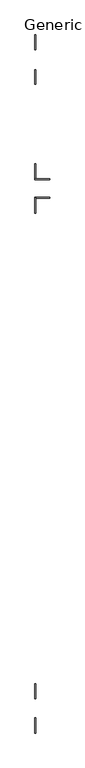
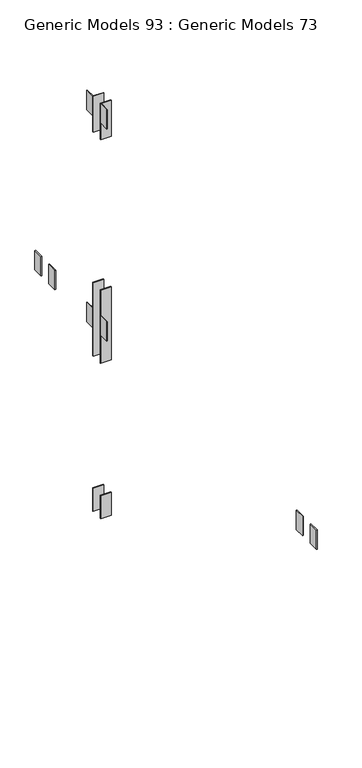
"""IFC4 building model written with IfcOpenShell, lengths in millimetres: proxy geometry, Generic Models 93 : Generic Models 73."""

import ifcopenshell
import ifcopenshell.guid

model = None  # the IFC model being written
_history = None  # IfcOwnerHistory: only IFC2X3 demands one
_inside = {}  # id of a spatial element -> (the spatial element, [elements in it])
_under = {}  # id of a project, library or spatial element -> (it, [spatial elements below it])
_declared = {}  # id of a project -> (the project, [libraries it declares])
_typed = {}  # id of a type object -> (the type object, [elements of that type])
_made_of = {}  # id of a material, layer set ... -> (it, [elements and type objects made of it])


def new_model(schema):
    """Start an empty IFC model of exactly this schema.

    Asked for "IFC4X3", IfcOpenShell would pick the latest addendum, in which some entities
    have other attributes; the version numbers below select the first issue.
    IFC2X3 requires an IfcOwnerHistory on every rooted entity: one is made here for all.
    """
    global model, _history
    if schema == "IFC4X3":
        model = ifcopenshell.file(schema_version=(4, 3, 0, 0))
    else:
        model = ifcopenshell.file(schema=schema)
    _inside.clear()
    _under.clear()
    _declared.clear()
    _typed.clear()
    _made_of.clear()
    _history = None
    if model.schema == "IFC2X3":
        org = make("IfcOrganization", Name="unknown")
        user = make(
            "IfcPersonAndOrganization",
            ThePerson=make("IfcPerson", FamilyName="unknown"),
            TheOrganization=org,
        )
        app = make(
            "IfcApplication",
            ApplicationDeveloper=org,
            Version="unknown",
            ApplicationFullName="unknown",
            ApplicationIdentifier="unknown",
        )
        _history = make(
            "IfcOwnerHistory",
            OwningUser=user,
            OwningApplication=app,
            ChangeAction="ADDED",
            CreationDate=0,
        )
    return model


def make(cls, **values):
    """One entity of the class cls with the attributes given. An attribute that is None is left unset."""
    return model.create_entity(
        cls, **{name: value for name, value in values.items() if value is not None}
    )


def rooted(cls, **values):
    """An entity with a GlobalId (a new one), such as an element, a storey or a relation."""
    return make(cls, GlobalId=ifcopenshell.guid.new(), OwnerHistory=_history, **values)


def si_unit(unit_type, name, prefix=None):
    """IfcSIUnit, for example si_unit("LENGTHUNIT", "METRE", prefix="MILLI")."""
    return make("IfcSIUnit", UnitType=unit_type, Prefix=prefix, Name=name)


def assignment(units):
    """IfcUnitAssignment: the units of a project."""
    return None if units is None else make("IfcUnitAssignment", Units=units)


def point(xyz):
    """IfcCartesianPoint."""
    return None if xyz is None else make("IfcCartesianPoint", Coordinates=xyz)


def direction(xyz):
    """IfcDirection."""
    return None if xyz is None else make("IfcDirection", DirectionRatios=xyz)


def frame(location, z_axis=None, x_axis=None):
    """IfcAxis2Placement3D, a coordinate frame: its origin and axes. An axis left out is left unset."""
    return make(
        "IfcAxis2Placement3D",
        Location=point(location),
        Axis=direction(z_axis),
        RefDirection=direction(x_axis),
    )


def origin():
    """The frame at (0, 0, 0) with its axes left unset."""
    return frame((0.0, 0.0, 0.0))


def place(relative_to, where):
    """IfcLocalPlacement: puts the frame where relative to a parent placement (None: the world)."""
    return make(
        "IfcLocalPlacement", PlacementRelTo=relative_to, RelativePlacement=where
    )


def context(
    kind, dimensions, precision=None, world=None, true_north=None, identifier=None
):
    """IfcGeometricRepresentationContext, for example the 3D "Model" context."""
    return make(
        "IfcGeometricRepresentationContext",
        ContextIdentifier=identifier,
        ContextType=kind,
        CoordinateSpaceDimension=dimensions,
        Precision=precision,
        WorldCoordinateSystem=world,
        TrueNorth=true_north,
    )


def project(units=None, contexts=None):
    """IfcProject with its units and contexts."""
    return rooted(
        "IfcProject",
        Name="project",
        RepresentationContexts=contexts,
        UnitsInContext=assignment(units),
    )


def spatial(cls, under=None, at=None, **own):
    """A site, building, storey or space (cls), placed at a placement, below another one or the project."""
    s = rooted(cls, ObjectPlacement=at, **own)
    if under is not None:
        _under.setdefault(under.id(), (under, []))[1].append(s)
    return s


def polyline(points):
    """IfcPolyline through the points."""
    return make("IfcPolyline", Points=[point(p) for p in points])


def outline(outer, holes=None, kind="AREA"):
    """IfcArbitraryClosedProfileDef: a profile drawn as a closed curve; with holes, ...WithVoids."""
    if holes is None:
        return make("IfcArbitraryClosedProfileDef", ProfileType=kind, OuterCurve=outer)
    return make(
        "IfcArbitraryProfileDefWithVoids",
        ProfileType=kind,
        OuterCurve=outer,
        InnerCurves=holes,
    )


def extrude(swept, where, along, depth):
    """IfcExtrudedAreaSolid: the profile swept, set in the frame where, extruded along a direction by depth."""
    return make(
        "IfcExtrudedAreaSolid",
        SweptArea=swept,
        Position=where,
        ExtrudedDirection=direction(along),
        Depth=depth,
    )


def shape(context_of_items, identifier, shape_type, items):
    """IfcShapeRepresentation: the items that make up one representation, for example the "Body"."""
    return make(
        "IfcShapeRepresentation",
        ContextOfItems=context_of_items,
        RepresentationIdentifier=identifier,
        RepresentationType=shape_type,
        Items=items,
    )


def source(mapping_origin, context_of_items, identifier, shape_type, items):
    """IfcRepresentationMap: a shape defined once, which mapped items show again and again."""
    return make(
        "IfcRepresentationMap",
        MappingOrigin=mapping_origin,
        MappedRepresentation=shape(context_of_items, identifier, shape_type, items),
    )


def transform(
    local_origin,
    x_axis=None,
    y_axis=None,
    z_axis=None,
    scale=None,
    scale2=None,
    scale3=None,
    uniform=True,
):
    """IfcCartesianTransformationOperator3D, or its non-uniform kind. x_axis, y_axis, z_axis: its Axis1, 2, 3."""
    if uniform:
        return make(
            "IfcCartesianTransformationOperator3D",
            Axis1=direction(x_axis),
            Axis2=direction(y_axis),
            LocalOrigin=point(local_origin),
            Scale=scale,
            Axis3=direction(z_axis),
        )
    return make(
        "IfcCartesianTransformationOperator3DnonUniform",
        Axis1=direction(x_axis),
        Axis2=direction(y_axis),
        LocalOrigin=point(local_origin),
        Scale=scale,
        Axis3=direction(z_axis),
        Scale2=scale2,
        Scale3=scale3,
    )


def mapped(mapping_source, mapping_target):
    """IfcMappedItem: shows the shape of a source again, moved by a transform."""
    return make(
        "IfcMappedItem", MappingSource=mapping_source, MappingTarget=mapping_target
    )


def made_of(thing, what):
    """Note that an element or type object is made of a material, layer set ...; save() writes the relation."""
    if what is not None:
        _made_of.setdefault(what.id(), (what, []))[1].append(thing)
    return thing


def element(
    cls,
    number,
    at=None,
    inside=None,
    cuts=None,
    type_object=None,
    material=None,
    context=None,
    identifier="Body",
    shape_type=None,
    held_by="IfcProductDefinitionShape",
    body=None,
    shapes=None,
    **own,
):
    """One element of the class cls, such as IfcWall. Its Tag is "e" and its number.

    at: its placement. inside: the storey or other place that contains it. cuts: it is an
    opening in that element (IfcRelVoidsElement). A single representation is given by context,
    identifier, shape_type and body (its items); several are given by shapes. held_by: the class
    of the entity that holds the representations. save() writes the other relations.
    """
    e = rooted(cls, Tag="e%d" % number, ObjectPlacement=at, **own)
    if body is not None:
        shapes = [shape(context, identifier, shape_type, body)]
    if shapes is not None:
        e.Representation = make(held_by, Representations=shapes)
    if inside is not None:
        _inside.setdefault(inside.id(), (inside, []))[1].append(e)
    if cuts is not None:
        rooted(
            "IfcRelVoidsElement", RelatingBuildingElement=cuts, RelatedOpeningElement=e
        )
    if type_object is not None:
        _typed.setdefault(type_object.id(), (type_object, []))[1].append(e)
    return made_of(e, material)


def aggregate(whole, parts):
    """IfcRelAggregates: a whole, such as a stair, and the parts it consists of."""
    return rooted("IfcRelAggregates", RelatingObject=whole, RelatedObjects=parts)


def save(model, path):
    """Write the relations noted so far, then the file.

    IfcRelAggregates (storeys below a building ...), IfcRelContainedInSpatialStructure (elements
    in a storey), IfcRelDefinesByType, IfcRelAssociatesMaterial and IfcRelDeclares: one each for
    every whole, place, type object, material and project.
    """
    for whole, parts in _under.values():
        aggregate(whole, parts)
    for where, things in _inside.values():
        rooted(
            "IfcRelContainedInSpatialStructure",
            RelatedElements=things,
            RelatingStructure=where,
        )
    for kind, things in _typed.values():
        rooted("IfcRelDefinesByType", RelatedObjects=things, RelatingType=kind)
    for what, things in _made_of.values():
        rooted("IfcRelAssociatesMaterial", RelatedObjects=things, RelatingMaterial=what)
    for by, libraries in _declared.values():
        rooted("IfcRelDeclares", RelatingContext=by, RelatedDefinitions=libraries)
    model.write(path)


def generic_models_93_generic_models_73_0b4a4ac0(model_context):
    return source(origin(), model_context, "Body", "SweptSolid", [
        extrude(outline(polyline([(31910.3221032, 30691.7906612), (31918.2596032, 30691.7906612), (31918.2596032, 30560.0281612), (31910.3221032, 30560.0281612), (31910.3221032, 30691.7906612)])), frame((0.0, 0.0, 268836.775), z_axis=(0.0, 0.0, 1.0), x_axis=(1.0, 0.0, 0.0)), (0.0, 0.0, 1.0), 254.0),
        extrude(outline(polyline([(31910.3221032, 30990.2406612), (31918.2596032, 30990.2406612), (31918.2596032, 30858.4781612), (31910.3221032, 30858.4781612), (31910.3221032, 30990.2406612)])), frame((0.0, 0.0, 268836.775), z_axis=(0.0, 0.0, 1.0), x_axis=(1.0, 0.0, 0.0)), (0.0, 0.0, 1.0), 254.0),
        extrude(outline(polyline([(31910.3221032, 36321.6957942), (31918.2596032, 36321.6957942), (31918.2596032, 36193.1082942), (31910.3221032, 36193.1082942), (31910.3221032, 36321.6957942)])), frame((0.0, 0.0, 268836.775), z_axis=(0.0, 0.0, 1.0), x_axis=(1.0, 0.0, 0.0)), (0.0, 0.0, 1.0), 254.0),
        extrude(outline(polyline([(31910.3221032, 36623.3207942), (31918.2596032, 36623.3207942), (31918.2596032, 36493.1457942), (31910.3221032, 36493.1457942), (31910.3221032, 36623.3207942)])), frame((0.0, 0.0, 268836.775), z_axis=(0.0, 0.0, 1.0), x_axis=(1.0, 0.0, 0.0)), (0.0, 0.0, 1.0), 254.0),
        extrude(outline(polyline([(31910.3221032, 35207.2707942), (31918.2596032, 35207.2707942), (31918.2596032, 35075.5082942), (31910.3221032, 35075.5082942), (31910.3221032, 35207.2707942)])), frame((0.0, 0.0, 271626.0125), z_axis=(0.0, 0.0, 1.0), x_axis=(1.0, 0.0, 0.0)), (0.0, 0.0, 1.0), 254.0),
        extrude(outline(polyline([(31910.3221032, 35505.7207942), (31918.2596032, 35505.7207942), (31918.2596032, 35373.9582942), (31910.3221032, 35373.9582942), (31910.3221032, 35505.7207942)])), frame((0.0, 0.0, 271621.25), z_axis=(0.0, 0.0, 1.0), x_axis=(1.0, 0.0, 0.0)), (0.0, 0.0, 1.0), 254.0),
        extrude(outline(polyline([(31910.3221032, 35207.2707942), (31918.2596032, 35207.2707942), (31918.2596032, 35075.5082942), (31910.3221032, 35075.5082942), (31910.3221032, 35207.2707942)])), frame((0.0, 0.0, 268836.775), z_axis=(0.0, 0.0, 1.0), x_axis=(1.0, 0.0, 0.0)), (0.0, 0.0, 1.0), 254.0),
        extrude(outline(polyline([(31910.3221032, 35505.7207942), (31918.2596032, 35505.7207942), (31918.2596032, 35373.9582942), (31910.3221032, 35373.9582942), (31910.3221032, 35505.7207942)])), frame((0.0, 0.0, 268832.0125), z_axis=(0.0, 0.0, 1.0), x_axis=(1.0, 0.0, 0.0)), (0.0, 0.0, 1.0), 254.0),
        extrude(outline(polyline([(32040.4971032, 35213.6207942), (32040.4971032, 35205.6832942), (31910.3221032, 35205.6832942), (31910.3221032, 35213.6207942), (32040.4971032, 35213.6207942)])), frame((0.0, 0.0, 266422.1875), z_axis=(0.0, 0.0, 1.0), x_axis=(1.0, 0.0, 0.0)), (0.0, 0.0, 1.0), 304.8),
        extrude(outline(polyline([(32040.4971032, 35373.9582942), (32040.4971032, 35366.0207942), (31910.3221032, 35366.0207942), (31910.3221032, 35373.9582942), (32040.4971032, 35373.9582942)])), frame((0.0, 0.0, 266422.1875), z_axis=(0.0, 0.0, 1.0), x_axis=(1.0, 0.0, 0.0)), (0.0, 0.0, 1.0), 304.8),
        extrude(outline(polyline([(32040.4971032, 35213.6207942), (32040.4971032, 35205.6832942), (31910.3221032, 35205.6832942), (31910.3221032, 35213.6207942), (32040.4971032, 35213.6207942)])), frame((0.0, 0.0, 271406.9375), z_axis=(0.0, 0.0, 1.0), x_axis=(1.0, 0.0, 0.0)), (0.0, 0.0, 1.0), 473.075),
        extrude(outline(polyline([(32040.4971032, 35373.9582942), (32040.4971032, 35366.0207942), (31910.3221032, 35366.0207942), (31910.3221032, 35373.9582942), (32040.4971032, 35373.9582942)])), frame((0.0, 0.0, 271406.9375), z_axis=(0.0, 0.0, 1.0), x_axis=(1.0, 0.0, 0.0)), (0.0, 0.0, 1.0), 473.075),
        extrude(outline(polyline([(32040.4971032, 35373.9582942), (32040.4971032, 35366.0207942), (31910.3221032, 35366.0207942), (31910.3221032, 35373.9582942), (32040.4971032, 35373.9582942)])), frame((0.0, 0.0, 268465.3), z_axis=(0.0, 0.0, 1.0), x_axis=(1.0, 0.0, 0.0)), (0.0, 0.0, 1.0), 965.2),
        extrude(outline(polyline([(32040.4971032, 35213.6207942), (32040.4971032, 35205.6832942), (31910.3221032, 35205.6832942), (31910.3221032, 35213.6207942), (32040.4971032, 35213.6207942)])), frame((0.0, 0.0, 268465.3), z_axis=(0.0, 0.0, 1.0), x_axis=(1.0, 0.0, 0.0)), (0.0, 0.0, 1.0), 965.2),
    ])


if __name__ == "__main__":
    model = new_model("IFC4")
    model_context = context("Model", 3, world=origin())
    ifc_project = project(units=[si_unit("LENGTHUNIT", "METRE", prefix="MILLI")], contexts=[model_context])
    site = spatial("IfcSite", under=ifc_project)
    building = spatial("IfcBuilding", under=site)
    placement = place(None, origin())
    generic_models_93_generic_models_73_shape = generic_models_93_generic_models_73_0b4a4ac0(model_context)
    element("IfcBuildingElementProxy", 1, Name="Generic Models 93 : Generic Models 73", ObjectType="Generic Models 93 : Generic Models 73", at=placement, inside=building, context=model_context, shape_type="MappedRepresentation", body=[
        mapped(generic_models_93_generic_models_73_shape, transform((0.0, 0.0, 0.0), x_axis=(1.0, 0.0, 0.0), y_axis=(0.0, 1.0, 0.0), z_axis=(0.0, 0.0, 1.0))),
    ])
    save(model, "model.ifc")

# Revit data of these elements
# Element 1 (IfcBuildingElementProxy, "Generic Models 93 : Generic Models 73")
#   Materials on its faces: "5 1/8 x 10 x 0 5/16\" PLATE W/ 3 1\"DIA. THRU BOLTS", "5/16 x 5 1/2\" x 1'-0\" SIDE PLATES  CAP\nW/ 2 3/4\"DIA. THRU BOLTS"
# Materials
#   "5 1/8 x 10 x 0 5/16\" PLATE W/ 3 1\"DIA. THRU BOLTS": class "Metal", colour RGB 199 199 199, transparency 0, Description = "Carbon steel", Cost = 0
#   "5/16 x 5 1/2\" x 1'-0\" SIDE PLATES  CAP\nW/ 2 3/4\"DIA. THRU BOLTS": class "Metal", colour RGB 199 199 199, transparency 0, Description = "Carbon steel", Cost = 0
